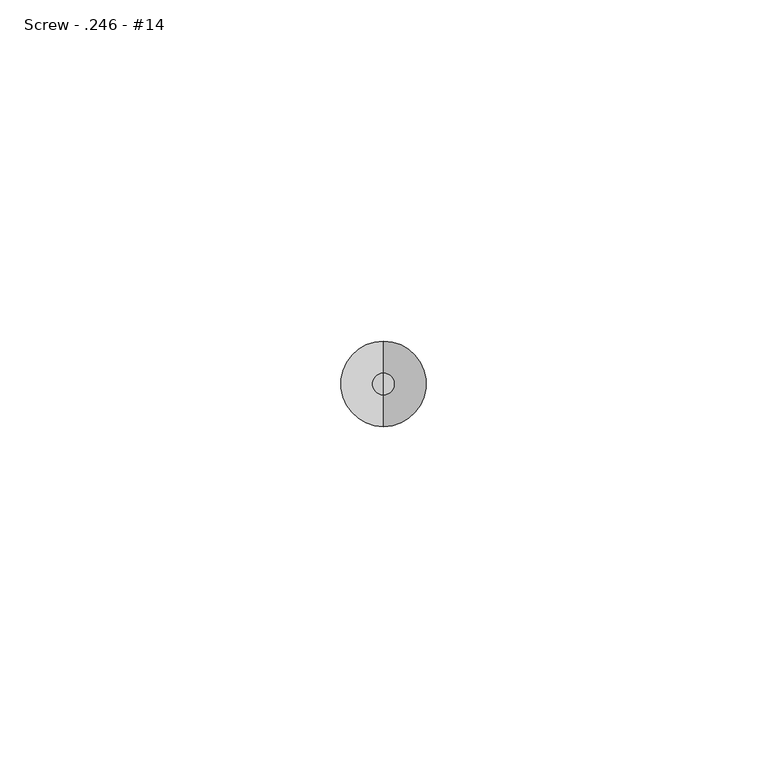
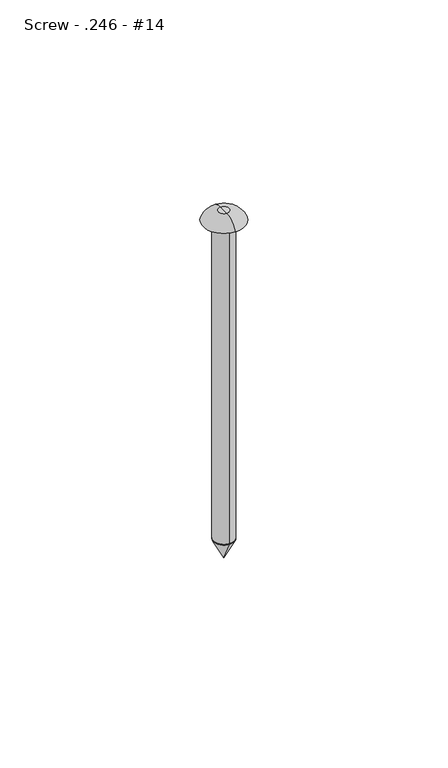
"""IFC4 building model written with IfcOpenShell, lengths in millimetres: fastener geometry, 060523 - W_P_C - Fastenings - Generic : Screw - .246 - #14."""

from ifc_helpers import new_model, si_unit, point, frame, origin, origin_2d, place, context, project, spatial, polyline, circle_curve, ellipse_curve, trimmed, segment, composite_curve, outline, extrude, source, transform, mapped, element, save
from ifc_brep_helpers import plane_surface, revolved_surface, advanced_brep


def screw_246_14_ceffc853(model_context):
    return source(origin(), model_context, "Body", "SolidModel", [
        advanced_brep(
        [(0.0, -3.1242, -101.6), (0.0, 3.1242, -101.6), (0.0, 0.0, -101.6), (0.0, 0.0, -107.8484)],
        [
            (0, 1, circle_curve(frame((0.0, 0.0, -101.6), z_axis=(0.0, 0.0, 1.0), x_axis=(0.0, 1.0, 0.0)), 3.1242)),
            (1, 2),
            (2, 0),
            (1, 0, circle_curve(frame((0.0, 0.0, -101.6), z_axis=(0.0, 0.0, 1.0), x_axis=(0.0, 1.0, 0.0)), 3.1242)),
            (3, 1),
            (0, 3),
        ],
        [
            plane_surface(frame((0.0, 0.0, -101.6), z_axis=(0.0, 0.0, 1.0), x_axis=(0.0, 1.0, 0.0))),
            revolved_surface(polyline([(0.0, 3.1242, -101.6), (0.0, 0.0, -107.8484)]), (0.0, 0.0, -103.0840259), (0.0, 0.0, -1.0)),
        ],
        [
            (0, [[1, 2, 3]]),
            (0, [[4, -3, -2]]),
            (1, [[5, -1, 6]]),
            (1, [[-6, -4, -5]]),
        ],
    ),
        advanced_brep(
        [(0.0, 6.2484, 0.0), (0.0, -6.2484, 0.0), (0.0, 0.0, 0.0), (0.0, 0.0, 3.1242), (0.0, -1.5875, 3.1242), (0.0, 1.5875, 3.1242)],
        [
            (0, 1, circle_curve(frame((0.0, 0.0, 0.0), z_axis=(0.0, 0.0, -1.0), x_axis=(0.0, -1.0, 0.0)), 6.2484)),
            (1, 2),
            (2, 0),
            (1, 0, circle_curve(frame((0.0, 0.0, 0.0), z_axis=(0.0, 0.0, -1.0), x_axis=(0.0, -1.0, 0.0)), 6.2484)),
            (3, 4),
            (4, 5, circle_curve(frame((0.0, 0.0, 3.1242), z_axis=(0.0, 0.0, 1.0), x_axis=(0.0, -1.0, 0.0)), 1.5875)),
            (5, 3),
            (5, 4, circle_curve(frame((0.0, 0.0, 3.1242), z_axis=(0.0, 0.0, 1.0), x_axis=(0.0, -1.0, 0.0)), 1.5875)),
            (4, 1, circle_curve(frame((0.0, -1.5875, -1.9146283), z_axis=(1.0, 0.0, 0.0), x_axis=(0.0, -1.0, 0.0)), 5.0388283)),
            (0, 5, circle_curve(frame((0.0, 1.5875, -1.9146283), z_axis=(1.0, 0.0, 0.0), x_axis=(0.0, 1.0, 0.0)), 5.0388283)),
        ],
        [
            plane_surface(frame((0.0, 0.0, 0.0), z_axis=(0.0, 0.0, -1.0), x_axis=(0.0, -1.0, 0.0))),
            plane_surface(frame((0.0, 0.0, 3.1242), z_axis=(0.0, 0.0, 1.0), x_axis=(0.0, -1.0, 0.0))),
            revolved_surface(trimmed(ellipse_curve(frame((0.0, -1.5875, -1.9146283), z_axis=(-1.0, 0.0, 0.0), x_axis=(0.0, -1.0, 0.0)), 5.0388283, 5.0388283), [point((0.0, -6.2484, 0.0))], [point((0.0, -1.5875, 3.1242))], True, "CARTESIAN"), (0.0, 0.0, 1.4840259), (0.0, 0.0, 1.0)),
        ],
        [
            (0, [[1, 2, 3]]),
            (0, [[4, -3, -2]]),
            (1, [[5, 6, 7]]),
            (1, [[-7, 8, -5]]),
            (2, [[-6, 9, -1, 10]]),
            (2, [[-8, -10, -4, -9]]),
        ],
    ),
        extrude(outline(composite_curve([segment(trimmed(circle_curve(origin_2d(), 3.1242), [point((0.0, -3.1242))], [point((0.0, 3.1242))], False, "CARTESIAN"), True, "CONTINUOUS"), segment(trimmed(circle_curve(origin_2d(), 3.1242), [point((0.0, 3.1242))], [point((0.0, -3.1242))], False, "CARTESIAN"), True, "CONTINUOUS")], self_intersect=False)), frame((0.0, 0.0, -101.6), z_axis=(0.0, 0.0, 1.0), x_axis=(1.0, 0.0, 0.0)), (0.0, 0.0, 1.0), 101.6),
    ])


if __name__ == "__main__":
    model = new_model("IFC4")
    model_context = context("Model", 3, world=origin())
    ifc_project = project(units=[si_unit("LENGTHUNIT", "METRE", prefix="MILLI")], contexts=[model_context])
    site = spatial("IfcSite", under=ifc_project)
    building = spatial("IfcBuilding", under=site)
    placement = place(None, origin())
    screw_246_14_shape = screw_246_14_ceffc853(model_context)
    element("IfcFastener", 1, ObjectType="060523 - W_P_C - Fastenings - Generic : Screw - .246 - #14", at=placement, inside=building, context=model_context, shape_type="MappedRepresentation", body=[
        mapped(screw_246_14_shape, transform((0.0, 0.0, 0.0), x_axis=(1.0, 0.0, 0.0), y_axis=(0.0, 1.0, 0.0), z_axis=(0.0, 0.0, 1.0))),
    ])
    save(model, "model.ifc")

# Revit data of these elements
# Type "060523 - W_P_C - Fastenings - Generic : Screw - .246 - #14"
#   Washer_Thickness = 0' - 0.00333"
#   Washer Radius = 0' - 0.133"
#   Washer Offset - Head = 0' - 0"
#   Washer Offset = 0' - 0"
#   Thickness_of_Substrate [instance default] = 0' - 1"
#   Side = 0' - 0 37/64"
#   Radius = 0' - 0.123"
#   Length [instance default] = 0' - 4"
#   Head Size = 0' - 1"
#   Head Radius = 0' - 0 1/2"
#   Head Height = 0' - 0.01"
#   Double Diameter = 0' - 0.492"
#   Diameter = 0' - 0.246"
#   Default Elevation = 4' - 0"
#   Washer_Nut_Visibility = no
#   Washer_Head_Visibility = no
#   Round_Head_Visibility = yes
#   Point Visibility = yes
#   Nut_Visibility = no
#   Hex_Head_Visiblilty = no
#   Washer Material = none
#   Bolt Material (Size) = AT SILL - FASTENER AT 24" O.C.
# Element 1 (IfcFastener, "060523 - W_P_C - Fastenings - Generic : Screw - .246 - #14")
#   Materials on its faces: "AT SILL - FASTENER AT 24\" O.C."
# Materials
#   "AT SILL - FASTENER AT 24\" O.C.": class "Generic", colour RGB 120 120 120, transparency 0, Cost = 0
